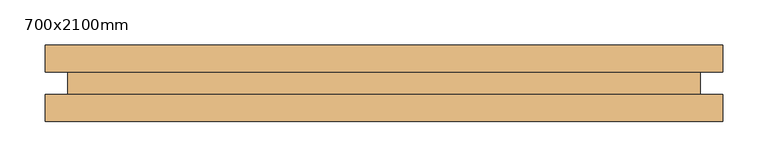
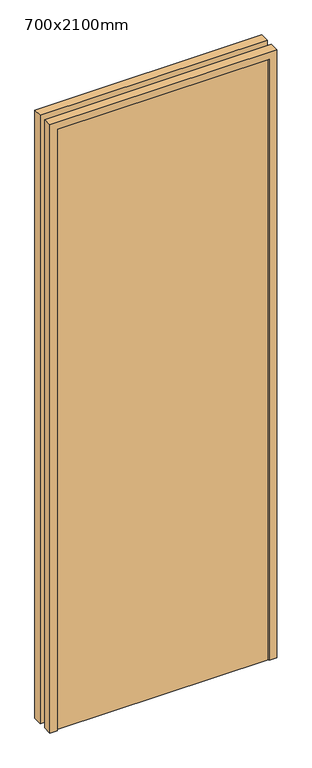
"""IFC4 building model written with IfcOpenShell, lengths in millimetres: door geometry, WWm-SingleSolid-Flush : 700x2100mm."""

from ifc_helpers import new_model, si_unit, frame, origin, origin_with_axes, place, context, project, spatial, polyline, outline, extrude, source, transform, mapped, element, save


def door_700x2100mm_7b2c5e55(model_context):
    return source(origin(), model_context, "Body", "SweptSolid", [
        extrude(outline(polyline([(2125.0, -375.0), (0.0, -375.0), (0.0, -350.0), (2100.0, -350.0), (2100.0, 350.0), (0.0, 350.0), (0.0, 375.0), (2125.0, 375.0), (2125.0, -375.0)])), frame((0.0, 12.5, 0.0), z_axis=(0.0, 1.0, 0.0), x_axis=(0.0, 0.0, 1.0)), (0.0, 0.0, 1.0), 30.0),
        extrude(outline(polyline([(2125.0, 375.0), (2125.0, -375.0), (0.0, -375.0), (0.0, -350.0), (2100.0, -350.0), (2100.0, 350.0), (0.0, 350.0), (0.0, 375.0), (2125.0, 375.0)])), frame((0.0, -42.5, 0.0), z_axis=(0.0, 1.0, 0.0), x_axis=(0.0, 0.0, 1.0)), (0.0, 0.0, 1.0), 30.0),
        extrude(outline(polyline([(350.0, -37.5), (-350.0, -37.5), (-350.0, 12.5), (350.0, 12.5), (350.0, -37.5)])), origin_with_axes(), (0.0, 0.0, 1.0), 2100.0),
    ])


if __name__ == "__main__":
    model = new_model("IFC4")
    model_context = context("Model", 3, world=origin())
    ifc_project = project(units=[si_unit("LENGTHUNIT", "METRE", prefix="MILLI")], contexts=[model_context])
    site = spatial("IfcSite", under=ifc_project)
    building = spatial("IfcBuilding", under=site)
    placement = place(None, origin())
    door_700x2100mm_shape = door_700x2100mm_7b2c5e55(model_context)
    element("IfcDoor", 1, ObjectType="WWm-SingleSolid-Flush : 700x2100mm", at=placement, inside=building, context=model_context, shape_type="MappedRepresentation", body=[
        mapped(door_700x2100mm_shape, transform((0.0, 0.0, 0.0), x_axis=(1.0, 0.0, 0.0), y_axis=(0.0, 1.0, 0.0), z_axis=(0.0, 0.0, 1.0))),
    ])
    save(model, "model.ifc")

# Revit data of these elements
# Type "WWm-SingleSolid-Flush : 700x2100mm"
#   Type Mark = "EX1-53"
#   Construction Type Id = "MDOOR"
#   Assembly Code = "C1020"
#   Analytic Construction = "Metal"
#   Thickness = 50 mm
#   Thermal Resistance (R) = 0.270117 (m²·K)/W
#   Heat Transfer Coefficient (U) = 3.7021 W/(m²·K)
#   Height = 2100 mm
#   Trim Projection Ext = 30 mm
#   Trim Projection Int = 30 mm
#   Trim Width = 25 mm
#   Width = 700 mm
#   Not 90 Degree [instance default] = no
#   90 Degree [instance default] = yes
#   Door Material = WW-EC-RGB-White
#   Frame Material = WW-EC-RGB-White
#   Visual Light Transmittance = 0
#   Solar Heat Gain Coefficient = 0
#   Function = (empty or 0)
#   Wall Closure = (empty or 0)
# Element 1 (IfcDoor, "WWm-SingleSolid-Flush : 700x2100mm")
#   Materials on its faces: "WW-EC-RGB-White"
# Materials
#   "WW-EC-RGB-White": class "Generic", colour RGB 255 255 255, transparency 0, Comments = "If region requests off-white, swith asset color to RGB 231-228-220", Description = "Generic Color", Cost = 0
